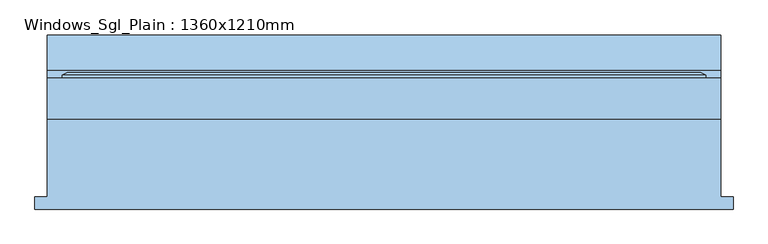
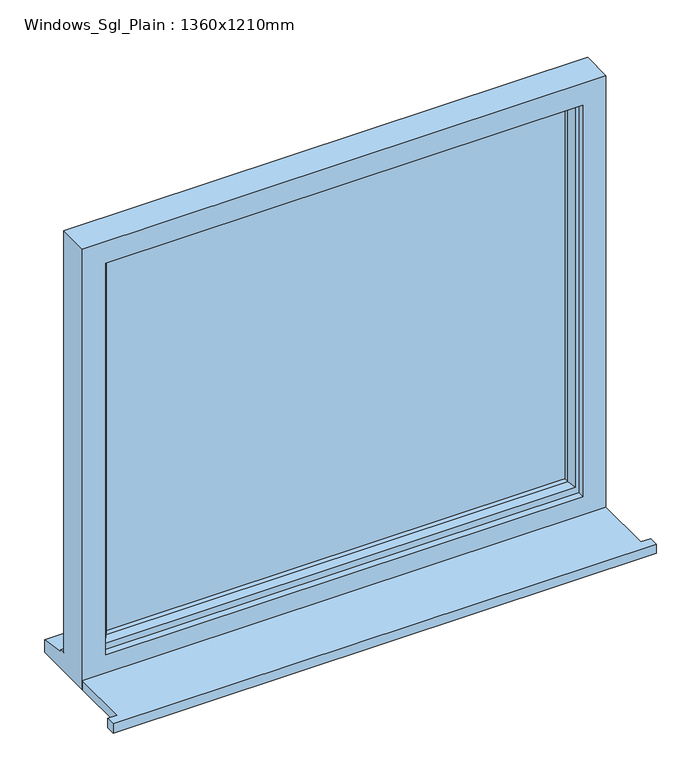
"""IFC4 building model written with IfcOpenShell, lengths in millimetres: window geometry, Windows_Sgl_Plain : 1360x1210mm."""

from ifc_helpers import new_model, si_unit, frame, origin, place, context, project, spatial, polyline, outline, extrude, faceted_brep, source, transform, mapped, element, save


def windows_sgl_plain_1360x1210mm_d0b87b97(model_context):
    return source(origin(), model_context, "Body", "SolidModel", [
        extrude(outline(polyline([(-705.0, -161.5434322), (-705.0, -136.5434322), (-680.0, -136.5434322), (-680.0, 20.4565678), (680.0, 20.4565678), (680.0, -136.5434322), (705.0, -136.5434322), (705.0, -161.5434322), (-705.0, -161.5434322)])), frame((0.0, 0.0, 900.0), z_axis=(0.0, 0.0, 1.0), x_axis=(1.0, 0.0, 0.0)), (0.0, 0.0, 1.0), 25.0),
        faceted_brep([(-680.0, 20.4565678, 900.0), (680.0, 20.4565678, 900.0), (680.0, 20.4565678, 2110.0), (-680.0, 20.4565678, 2110.0), (-620.0, 20.4565678, 2050.0), (620.0, 20.4565678, 2050.0), (620.0, 20.4565678, 975.0), (-620.0, 20.4565678, 975.0), (-680.0, 103.4565678, 2110.0), (-680.0, 103.4565678, 951.0), (-680.0, 118.4565678, 949.68767), (-680.0, 118.4565678, 944.7449676), (-680.0, 190.9565678, 933.8088847), (-680.0, 190.9565678, 900.0), (680.0, 103.4565678, 2110.0), (680.0, 103.4565678, 951.0), (-640.0, 103.4565678, 2070.0), (-640.0, 103.4565678, 963.0), (640.0, 103.4565678, 963.0), (640.0, 103.4565678, 2070.0), (-640.0, 38.4565678, 2070.0), (-640.0, 38.4565678, 963.0), (640.0, 38.4565678, 2070.0), (640.0, 38.4565678, 963.0), (-620.0, 38.4565678, 2050.0), (-620.0, 38.4565678, 975.0), (620.0, 38.4565678, 975.0), (620.0, 38.4565678, 2050.0), (680.0, 190.9565678, 900.0), (680.0, 190.9565678, 933.8088847), (680.0, 118.4565678, 944.7449676), (680.0, 118.4565678, 949.68767)], [[[0, 1, 2, 3], [4, 5, 6, 7]], [[0, 3, 8, 9, 10, 11, 12, 13]], [[9, 8, 14, 15], [16, 17, 18, 19]], [[17, 16, 20, 21]], [[20, 22, 23, 21], [24, 25, 26, 27]], [[24, 4, 7, 25]], [[3, 2, 14, 8]], [[16, 19, 22, 20]], [[5, 4, 24, 27]], [[15, 14, 2, 1, 28, 29, 30, 31]], [[19, 18, 23, 22]], [[5, 27, 26, 6]], [[28, 1, 0, 13]], [[29, 28, 13, 12]], [[30, 29, 12, 11]], [[31, 30, 11, 10]], [[15, 31, 10, 9]], [[21, 23, 18, 17]], [[7, 6, 26, 25]]]),
        extrude(outline(polyline([(610.0, 67.4565678), (-610.0, 67.4565678), (-610.0, 91.4565678), (610.0, 91.4565678), (610.0, 67.4565678)])), frame((0.0, 0.0, 993.0), z_axis=(0.0, 0.0, 1.0), x_axis=(1.0, 0.0, 0.0)), (0.0, 0.0, 1.0), 1047.0),
        faceted_brep([(-650.0, 103.4565678, 2080.0), (-650.0, 109.2300705, 2080.0), (-650.0, 109.2300705, 953.0), (-650.0, 103.4565678, 953.0), (-640.0, 38.4565678, 2070.0), (-640.0, 103.4565678, 2070.0), (-640.0, 103.4565678, 963.0), (-640.0, 38.4565678, 963.0), (-600.0, 52.9494677, 2030.0), (-610.1480377, 38.4565678, 2040.1480377), (-610.1480377, 38.4565678, 992.8519623), (-600.0, 52.9494677, 1003.0), (-600.0, 67.4565678, 2030.0), (-600.0, 67.4565678, 1003.0), (-610.0, 91.4565678, 2040.0), (-610.0, 67.4565678, 2040.0), (-610.0, 67.4565678, 993.0), (-610.0, 91.4565678, 993.0), (-600.0, 109.2300705, 2030.0), (-600.0, 91.4565678, 2030.0), (-600.0, 91.4565678, 1003.0), (-600.0, 109.2300705, 1003.0), (-617.4457548, 115.0035732, 2047.4457548), (-617.4457548, 115.0035732, 985.5542452), (-639.2153903, 115.0035732, 2069.2153903), (-639.2153903, 115.0035732, 963.7846097), (650.0, 109.2300705, 953.0), (650.0, 103.4565678, 953.0), (640.0, 103.4565678, 963.0), (640.0, 38.4565678, 963.0), (610.1480377, 38.4565678, 992.8519623), (600.0, 52.9494677, 1003.0), (600.0, 67.4565678, 1003.0), (610.0, 67.4565678, 993.0), (610.0, 91.4565678, 993.0), (600.0, 91.4565678, 1003.0), (600.0, 109.2300705, 1003.0), (617.4457548, 115.0035732, 985.5542452), (639.2153903, 115.0035732, 963.7846097), (650.0, 109.2300705, 2080.0), (650.0, 103.4565678, 2080.0), (640.0, 103.4565678, 2070.0), (640.0, 38.4565678, 2070.0), (610.1480377, 38.4565678, 2040.1480377), (600.0, 52.9494677, 2030.0), (600.0, 67.4565678, 2030.0), (610.0, 67.4565678, 2040.0), (610.0, 91.4565678, 2040.0), (600.0, 91.4565678, 2030.0), (600.0, 109.2300705, 2030.0), (617.4457548, 115.0035732, 2047.4457548), (639.2153903, 115.0035732, 2069.2153903)], [[[0, 1, 2, 3]], [[4, 5, 6, 7]], [[8, 9, 10, 11]], [[12, 8, 11, 13]], [[14, 15, 16, 17]], [[18, 19, 20, 21]], [[22, 18, 21, 23]], [[1, 24, 25, 2]], [[3, 2, 26, 27]], [[7, 6, 28, 29]], [[11, 10, 30, 31]], [[13, 11, 31, 32]], [[17, 16, 33, 34]], [[21, 20, 35, 36]], [[23, 21, 36, 37]], [[2, 25, 38, 26]], [[27, 26, 39, 40]], [[29, 28, 41, 42]], [[31, 30, 43, 44]], [[32, 31, 44, 45]], [[34, 33, 46, 47]], [[36, 35, 48, 49]], [[37, 36, 49, 50]], [[26, 38, 51, 39]], [[40, 39, 1, 0]], [[3, 27, 40, 0], [5, 41, 28, 6]], [[42, 41, 5, 4]], [[7, 29, 42, 4], [9, 43, 30, 10]], [[44, 43, 9, 8]], [[45, 44, 8, 12]], [[15, 46, 33, 16], [13, 32, 45, 12]], [[47, 46, 15, 14]], [[17, 34, 47, 14], [19, 48, 35, 20]], [[49, 48, 19, 18]], [[50, 49, 18, 22]], [[24, 51, 38, 25], [23, 37, 50, 22]], [[39, 51, 24, 1]]]),
    ])


if __name__ == "__main__":
    model = new_model("IFC4")
    model_context = context("Model", 3, world=origin())
    ifc_project = project(units=[si_unit("LENGTHUNIT", "METRE", prefix="MILLI")], contexts=[model_context])
    site = spatial("IfcSite", under=ifc_project)
    building = spatial("IfcBuilding", under=site)
    placement = place(None, origin())
    windows_sgl_plain_1360x1210mm_shape = windows_sgl_plain_1360x1210mm_d0b87b97(model_context)
    element("IfcWindow", 1, ObjectType="Windows_Sgl_Plain : 1360x1210mm", at=placement, inside=building, context=model_context, shape_type="MappedRepresentation", body=[
        mapped(windows_sgl_plain_1360x1210mm_shape, transform((0.0, 0.0, 0.0), x_axis=(1.0, 0.0, 0.0), y_axis=(0.0, 1.0, 0.0), z_axis=(0.0, 0.0, 1.0))),
    ])
    save(model, "model.ifc")

# Revit data of these elements
# Type "Windows_Sgl_Plain : 1360x1210mm"
#   Type Mark = "47"
#   Operation = "SinglePanel"
#   Construction Type Id = "SGL"
#   Manufacturer = "Revit"
#   Keynote = "L10"
#   Analytic Construction = "Large single-glazed windows"
#   Wrap Layers (Ext) from Ext = 102.5 mm
#   Wrap Layers (Int) from Ext = 177.5 mm
#   Window Board Projection = 25 mm
#   Window Board Extension = 25 mm
#   Visual Light Transmittance = 0.9
#   Solar Heat Gain Coefficient = 0.86
#   Rough Width = 1360 mm
#   Rough Height = 1210 mm
#   Height = 1210 mm
#   Width = 1360 mm
#   Heat Transfer Coefficient (U) = 5.5617 W/(m²·K)
#   Glazing Thickness = 24 mm
#   FrameOffset - External = 50 mm
#   Frame Depth = 65 mm
#   Default Head Height = 2110 mm
#   Cill Depth = 87.5 mm
#   Cavity Closer Width = 50 mm
#   Cavity Closer Offset from Ext = 102.5 mm
#   Cavity Closer Depth = 85 mm
#   Define Thermal Properties by = 1
#   Vis - Cavity Closers = yes
#   Define Thermal Properties by = 1
#   Material Trim = Window Frame
#   Material Glass = Glass
#   Material Frame = Window Frame
#   Wall Closure = (empty or 0)
# Element 1 (IfcWindow, "Windows_Sgl_Plain : 1360x1210mm")
#   Materials on its faces: "Window Frame", "Glass"
# Materials
#   "Window Frame": class "Miscellaneous", colour RGB 249 249 249, transparency 0, Keynote = "L10", Cost = 0
#   "Glass": class "Glass", colour RGB 0 128 192, transparency 0.9, Description = "Soda Lime Glass", Cost = 0
